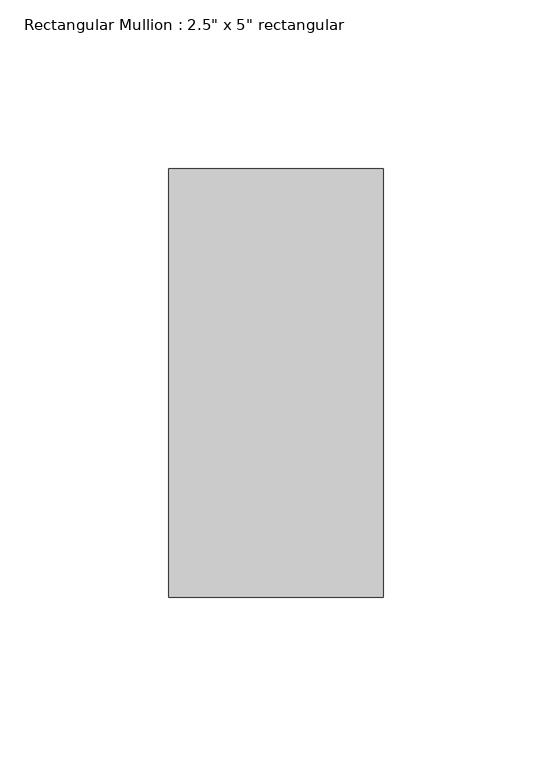
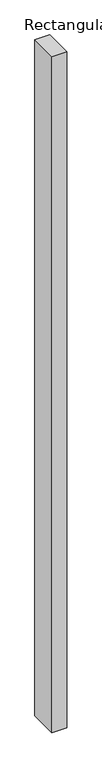
"""IFC4 building model written with IfcOpenShell, lengths in millimetres: member geometry."""

from ifc_helpers import new_model, si_unit, frame, origin, place, context, project, spatial, polyline, outline, extrude, source, transform, mapped, element, save


def member_e8b2a95c(model_context):
    return source(origin(), model_context, "Body", "SweptSolid", [
        extrude(outline(polyline([(0.0, 63.5), (0.0, -63.5), (-63.5, -63.5), (-63.5, 63.5), (0.0, 63.5)])), frame((0.0, 0.0, -3086.1), z_axis=(0.0, 0.0, 1.0), x_axis=(1.0, 0.0, 0.0)), (0.0, 0.0, 1.0), 3086.1),
    ])


if __name__ == "__main__":
    model = new_model("IFC4")
    model_context = context("Model", 3, world=origin())
    ifc_project = project(units=[si_unit("LENGTHUNIT", "METRE", prefix="MILLI")], contexts=[model_context])
    site = spatial("IfcSite", under=ifc_project)
    building = spatial("IfcBuilding", under=site)
    placement = place(None, origin())
    member_shape = member_e8b2a95c(model_context)
    element("IfcMember", 1, ObjectType="Rectangular Mullion : 2.5\" x 5\" rectangular", at=placement, inside=building, context=model_context, shape_type="MappedRepresentation", body=[
        mapped(member_shape, transform((0.0, 0.0, 0.0), x_axis=(1.0, 0.0, 0.0), y_axis=(0.0, 1.0, 0.0), z_axis=(0.0, 0.0, 1.0))),
    ])
    save(model, "model.ifc")

# Revit data of these elements
# Type "Rectangular Mullion : 2.5\" x 5\" rectangular"
#   built-in parameter 1007304 = 0.416667 (stored number, unit not read)
#   built-in parameter 1007301 = 0.104167 (stored number, unit not read)
#   built-in parameter 1007300 = 0.104167 (stored number, unit not read)
# Element 1 (IfcMember, "Rectangular Mullion : 2.5\" x 5\" rectangular")
#   Materials on its faces: "Aluminum"
# Materials
#   "Aluminum": class "Metal", colour RGB 247 247 247, transparency 0, Description = "Aluminum 6061", Cost = 0
